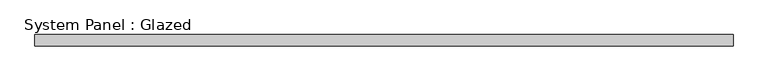
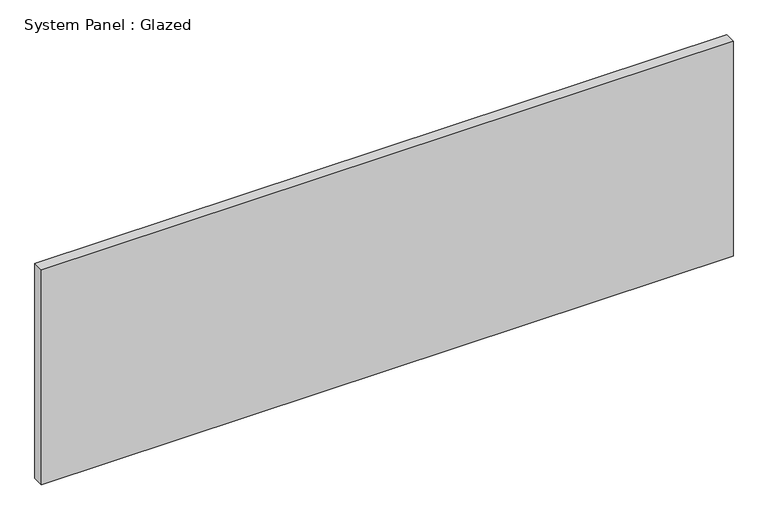
"""IFC4 building model written with IfcOpenShell, lengths in millimetres: plate geometry, System Panel : Glazed."""

from ifc_helpers import new_model, si_unit, origin, origin_with_axes, place, context, project, spatial, polyline, outline, extrude, source, transform, mapped, element, save


def system_panel_glazed_1f8eab1a(model_context):
    return source(origin(), model_context, "Body", "SweptSolid", [
        extrude(outline(polyline([(769.3237049, 24.5), (-769.3237049, 24.5), (-769.3237049, 49.5), (769.3237049, 49.5), (769.3237049, 24.5)])), origin_with_axes(), (0.0, 0.0, 1.0), 505.0),
    ])


if __name__ == "__main__":
    model = new_model("IFC4")
    model_context = context("Model", 3, world=origin())
    ifc_project = project(units=[si_unit("LENGTHUNIT", "METRE", prefix="MILLI")], contexts=[model_context])
    site = spatial("IfcSite", under=ifc_project)
    building = spatial("IfcBuilding", under=site)
    placement = place(None, origin())
    system_panel_glazed_shape = system_panel_glazed_1f8eab1a(model_context)
    element("IfcPlate", 1, ObjectType="System Panel : Glazed", at=placement, inside=building, context=model_context, shape_type="MappedRepresentation", body=[
        mapped(system_panel_glazed_shape, transform((0.0, 0.0, 0.0), x_axis=(1.0, 0.0, 0.0), y_axis=(0.0, 1.0, 0.0), z_axis=(0.0, 0.0, 1.0))),
    ])
    save(model, "model.ifc")

# Revit data of these elements
# Element 1 (IfcPlate, "System Panel : Glazed")
#   Materials on its faces: "Glass"
# Materials
#   "Glass": class "Glass", colour RGB 218 227 224, transparency 0.85, Description = "Soda Lime Glass", Cost = 0
